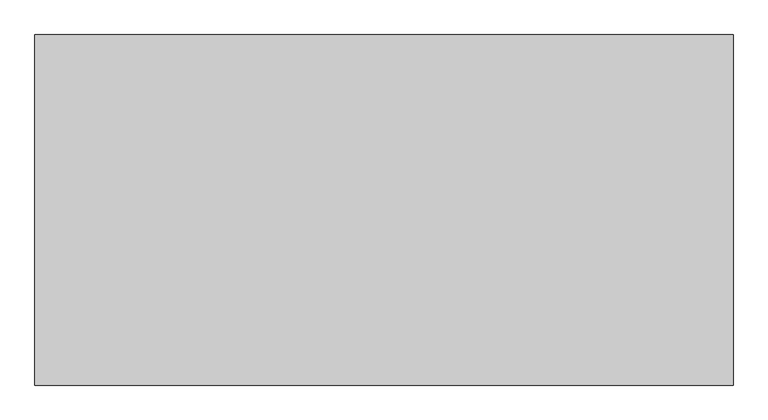
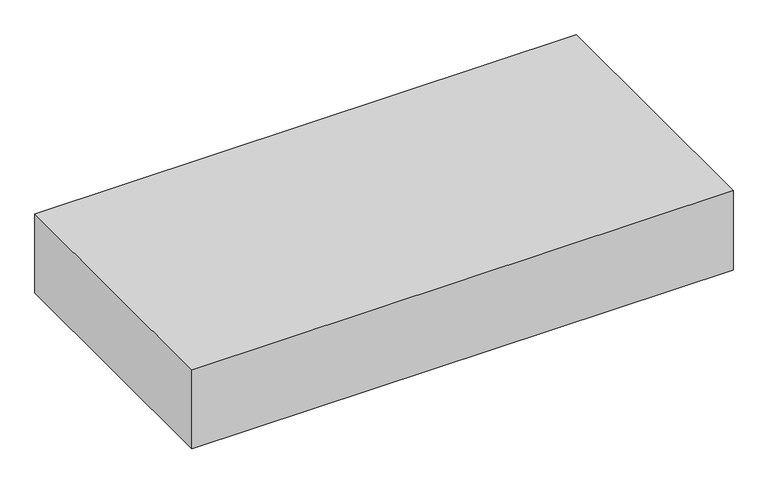
"""IFC4 building model written with IfcOpenShell, lengths in millimetres: proxy geometry, Fensteröffnung."""

from ifc_helpers import new_model, si_unit, origin, origin_with_axes, place, context, project, spatial, polyline, outline, extrude, source, transform, mapped, element, save


def generic_models_890812fe(model_context):
    return source(origin(), model_context, "Body", "SweptSolid", [
        extrude(outline(polyline([(0.0, 0.0), (0.0, 1135.0), (2260.0, 1135.0), (2260.0, 0.0), (0.0, 0.0)])), origin_with_axes(), (0.0, 0.0, 1.0), 350.0),
    ])


if __name__ == "__main__":
    model = new_model("IFC4")
    model_context = context("Model", 3, world=origin())
    ifc_project = project(units=[si_unit("LENGTHUNIT", "METRE", prefix="MILLI")], contexts=[model_context])
    site = spatial("IfcSite", under=ifc_project)
    building = spatial("IfcBuilding", under=site)
    placement = place(None, origin())
    generic_models_shape = generic_models_890812fe(model_context)
    element("IfcBuildingElementProxy", 1, Name="Fensteröffnung", ObjectType="Fensteröffnung", at=placement, inside=building, context=model_context, shape_type="MappedRepresentation", body=[
        mapped(generic_models_shape, transform((0.0, 0.0, 0.0), x_axis=(1.0, 0.0, 0.0), y_axis=(0.0, 1.0, 0.0), z_axis=(0.0, 0.0, 1.0))),
    ])
    save(model, "model.ifc")

# Revit data of these elements
# Element 1 (IfcBuildingElementProxy, "Fensteröffnung")
#   Materials on its faces: "IfcOpeningElement"
# Materials
#   "IfcOpeningElement": class "Unassigned", colour RGB 255 165 0, transparency 0.75
